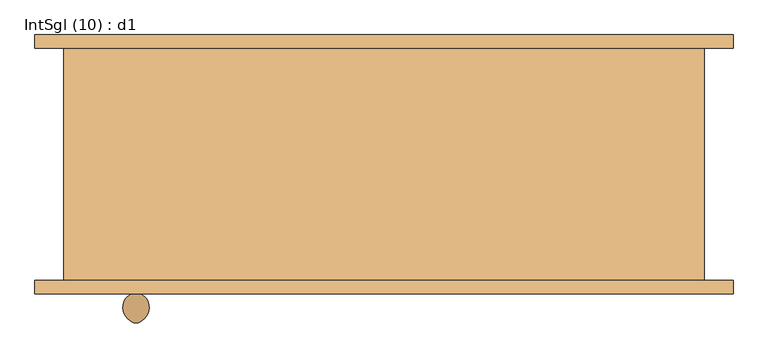
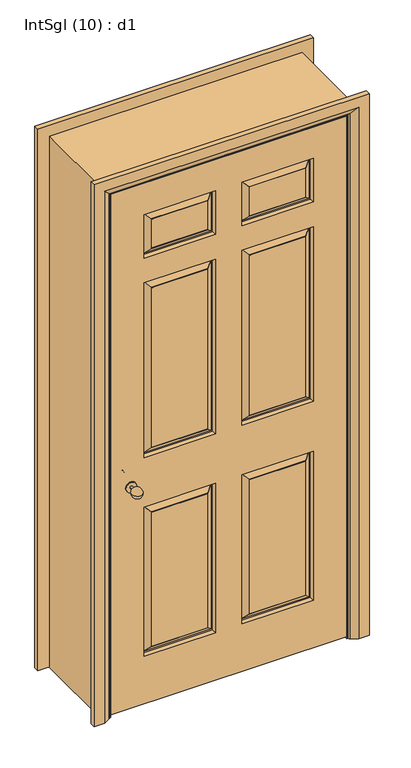
"""IFC4 building model written with IfcOpenShell, lengths in millimetres: door geometry, IntSgl (10) : d1."""

from ifc_helpers import new_model, si_unit, point, frame, origin, place, context, project, spatial, polyline, circle_curve, ellipse_curve, trimmed, outline, extrude, faceted_brep, source, transform, mapped, element, save
from ifc_brep_helpers import plane_surface, cylinder_surface, revolved_surface, advanced_brep


def intsgl_10_d1_80eab747(model_context):
    return source(origin(), model_context, "Body", "SolidModel", [
        advanced_brep(
        [(-368.0, -118.0, 900.0), (-378.0, -118.0, 900.0), (-373.0, -73.562589, 900.0), (-368.0, -133.0, 900.0), (-378.0, -133.0, 900.0), (-393.0, -137.0, 900.0), (-353.0, -137.0, 900.0), (-393.0, -133.0, 900.0), (-353.0, -133.0, 900.0)],
        [
            (0, 1, circle_curve(frame((-373.0, -118.0, 900.0), z_axis=(0.0, 1.0, 0.0), x_axis=(-1.0, 0.0, 0.0)), 5.0)),
            (1, 2, circle_curve(frame((-369.8115138, -96.4213505, 900.0), z_axis=(0.0, 0.0, -1.0), x_axis=(0.0, -1.0, 0.0)), 23.0800654)),
            (2, 0, circle_curve(frame((-376.1884862, -96.4213505, 900.0), z_axis=(0.0, 0.0, -1.0), x_axis=(0.0, -1.0, 0.0)), 23.0800654)),
            (1, 0, circle_curve(frame((-373.0, -118.0, 900.0), z_axis=(0.0, 1.0, 0.0), x_axis=(-1.0, 0.0, 0.0)), 5.0)),
            (0, 3),
            (3, 4, circle_curve(frame((-373.0, -133.0, 900.0), z_axis=(0.0, 1.0, 0.0), x_axis=(-1.0, 0.0, 0.0)), 5.0)),
            (4, 1),
            (4, 3, circle_curve(frame((-373.0, -133.0, 900.0), z_axis=(0.0, 1.0, 0.0), x_axis=(-1.0, 0.0, 0.0)), 5.0)),
            (5, 6, circle_curve(frame((-373.0, -137.0, 900.0), z_axis=(0.0, -1.0, 0.0), x_axis=(1.0, 0.0, 0.0)), 20.0)),
            (6, 5, circle_curve(frame((-373.0, -137.0, 900.0), z_axis=(0.0, -1.0, 0.0), x_axis=(1.0, 0.0, 0.0)), 20.0)),
            (7, 8, circle_curve(frame((-373.0, -133.0, 900.0), z_axis=(0.0, 1.0, 0.0), x_axis=(1.0, 0.0, 0.0)), 20.0)),
            (8, 7, circle_curve(frame((-373.0, -133.0, 900.0), z_axis=(0.0, 1.0, 0.0), x_axis=(1.0, 0.0, 0.0)), 20.0)),
            (5, 7),
            (8, 6),
        ],
        [
            revolved_surface(trimmed(ellipse_curve(frame((-369.8115138, -96.4213505, 900.0), z_axis=(0.0, 0.0, 1.0), x_axis=(0.0, -1.0, 0.0)), 23.0800654, 23.0800654), [point((-373.0, -73.562589, 900.0))], [point((-378.0, -118.0, 900.0))], True, "CARTESIAN"), (-373.0, -133.0, 900.0), (0.0, -1.0, 0.0)),
            cylinder_surface(frame((-373.0, -133.0, 900.0), z_axis=(0.0, -1.0, 0.0), x_axis=(-1.0, 0.0, 0.0)), 5.0),
            plane_surface(frame((-353.0, -137.0, 900.0), z_axis=(0.0, -1.0, 0.0), x_axis=(0.0, 0.0, 1.0))),
            plane_surface(frame((-353.0, -133.0, 900.0), z_axis=(0.0, 1.0, 0.0), x_axis=(0.0, 0.0, -1.0))),
            cylinder_surface(frame((-373.0, -133.0, 900.0), z_axis=(0.0, -1.0, 0.0), x_axis=(1.0, 0.0, 0.0)), 20.0),
        ],
        [
            (0, [[1, 2, 3]]),
            (0, [[-2, 4, -3]]),
            (1, [[-1, 5, 6, 7]]),
            (1, [[-4, -7, 8, -5]]),
            (2, [[9, 10]]),
            (3, [[11, 12], [-6, -8]]),
            (4, [[-9, 13, -12, 14]]),
            (4, [[-10, -14, -11, -13]]),
        ],
    ),
        advanced_brep(
        [(-368.0, -194.0, 900.0), (-373.0, -238.437411, 900.0), (-378.0, -194.0, 900.0), (-378.0, -179.0, 900.0), (-368.0, -179.0, 900.0), (-393.0, -175.0, 900.0), (-353.0, -175.0, 900.0), (-393.0, -179.0, 900.0), (-353.0, -179.0, 900.0)],
        [
            (0, 1, circle_curve(frame((-376.1884862, -215.5786495, 900.0), z_axis=(0.0, 0.0, -1.0), x_axis=(0.0, 1.0, 0.0)), 23.0800654)),
            (1, 2, circle_curve(frame((-369.8115138, -215.5786495, 900.0), z_axis=(0.0, 0.0, -1.0), x_axis=(0.0, 1.0, 0.0)), 23.0800654)),
            (2, 0, circle_curve(frame((-373.0, -194.0, 900.0), z_axis=(0.0, -1.0, 0.0), x_axis=(-1.0, 0.0, 0.0)), 5.0)),
            (0, 2, circle_curve(frame((-373.0, -194.0, 900.0), z_axis=(0.0, -1.0, 0.0), x_axis=(-1.0, 0.0, 0.0)), 5.0)),
            (2, 3),
            (3, 4, circle_curve(frame((-373.0, -179.0, 900.0), z_axis=(0.0, -1.0, 0.0), x_axis=(-1.0, 0.0, 0.0)), 5.0)),
            (4, 0),
            (4, 3, circle_curve(frame((-373.0, -179.0, 900.0), z_axis=(0.0, -1.0, 0.0), x_axis=(-1.0, 0.0, 0.0)), 5.0)),
            (5, 6, circle_curve(frame((-373.0, -175.0, 900.0), z_axis=(0.0, 1.0, 0.0), x_axis=(1.0, 0.0, 0.0)), 20.0)),
            (6, 5, circle_curve(frame((-373.0, -175.0, 900.0), z_axis=(0.0, 1.0, 0.0), x_axis=(1.0, 0.0, 0.0)), 20.0)),
            (7, 8, circle_curve(frame((-373.0, -179.0, 900.0), z_axis=(0.0, -1.0, 0.0), x_axis=(1.0, 0.0, 0.0)), 20.0)),
            (8, 7, circle_curve(frame((-373.0, -179.0, 900.0), z_axis=(0.0, -1.0, 0.0), x_axis=(1.0, 0.0, 0.0)), 20.0)),
            (6, 8),
            (7, 5),
        ],
        [
            revolved_surface(trimmed(ellipse_curve(frame((-369.8115138, -215.5786495, 900.0), z_axis=(0.0, 0.0, -1.0), x_axis=(0.0, 1.0, 0.0)), 23.0800654, 23.0800654), [point((-373.0, -238.437411, 900.0))], [point((-378.0, -194.0, 900.0))], True, "CARTESIAN"), (-373.0, -179.0, 900.0), (0.0, 1.0, 0.0)),
            cylinder_surface(frame((-373.0, -179.0, 900.0), z_axis=(0.0, 1.0, 0.0), x_axis=(-1.0, 0.0, 0.0)), 5.0),
            plane_surface(frame((-353.0, -175.0, 900.0), z_axis=(0.0, 1.0, 0.0), x_axis=(0.0, 0.0, 1.0))),
            plane_surface(frame((-353.0, -179.0, 900.0), z_axis=(0.0, -1.0, 0.0), x_axis=(0.0, 0.0, -1.0))),
            cylinder_surface(frame((-373.0, -179.0, 900.0), z_axis=(0.0, 1.0, 0.0), x_axis=(1.0, 0.0, 0.0)), 20.0),
        ],
        [
            (0, [[1, 2, 3]]),
            (0, [[-1, 4, -2]]),
            (1, [[5, 6, 7, -3]]),
            (1, [[-7, 8, -5, -4]]),
            (2, [[9, 10]]),
            (3, [[11, 12], [-8, -6]]),
            (4, [[13, -11, 14, -10]]),
            (4, [[-14, -12, -13, -9]]),
        ],
    ),
        faceted_brep([(-448.0, -137.0, 2103.0), (448.0, -137.0, 2103.0), (448.0, -137.0, 8.0), (-448.0, -137.0, 8.0), (-50.0, -137.0, 800.0), (-323.0, -137.0, 800.0), (-323.0, -137.0, 200.0), (-50.0, -137.0, 200.0), (323.0, -137.0, 800.0), (50.0, -137.0, 800.0), (50.0, -137.0, 200.0), (323.0, -137.0, 200.0), (-50.0, -137.0, 1703.0), (-323.0, -137.0, 1703.0), (-323.0, -137.0, 1000.0), (-50.0, -137.0, 1000.0), (323.0, -137.0, 1703.0), (50.0, -137.0, 1703.0), (50.0, -137.0, 1000.0), (323.0, -137.0, 1000.0), (-50.0, -137.0, 1978.0), (-323.0, -137.0, 1978.0), (-323.0, -137.0, 1803.0), (-50.0, -137.0, 1803.0), (323.0, -137.0, 1978.0), (50.0, -137.0, 1978.0), (50.0, -137.0, 1803.0), (323.0, -137.0, 1803.0), (-80.0, -137.0, 230.0), (-293.0, -137.0, 230.0), (-293.0, -137.0, 770.0), (-80.0, -137.0, 770.0), (293.0, -137.0, 230.0), (80.0, -137.0, 230.0), (80.0, -137.0, 770.0), (293.0, -137.0, 770.0), (-80.0, -137.0, 1030.0), (-293.0, -137.0, 1030.0), (-293.0, -137.0, 1673.0), (-80.0, -137.0, 1673.0), (293.0, -137.0, 1030.0), (80.0, -137.0, 1030.0), (80.0, -137.0, 1673.0), (293.0, -137.0, 1673.0), (-80.0, -137.0, 1833.0), (-293.0, -137.0, 1833.0), (-293.0, -137.0, 1948.0), (-80.0, -137.0, 1948.0), (293.0, -137.0, 1833.0), (80.0, -137.0, 1833.0), (80.0, -137.0, 1948.0), (293.0, -137.0, 1948.0), (-448.0, -175.0, 2103.0), (-448.0, -175.0, 8.0), (448.0, -175.0, 8.0), (448.0, -175.0, 2103.0), (50.0, -175.0, 800.0), (323.0, -175.0, 800.0), (323.0, -175.0, 200.0), (50.0, -175.0, 200.0), (-323.0, -175.0, 800.0), (-50.0, -175.0, 800.0), (-50.0, -175.0, 200.0), (-323.0, -175.0, 200.0), (50.0, -175.0, 1703.0), (323.0, -175.0, 1703.0), (323.0, -175.0, 1000.0), (50.0, -175.0, 1000.0), (-323.0, -175.0, 1703.0), (-50.0, -175.0, 1703.0), (-50.0, -175.0, 1000.0), (-323.0, -175.0, 1000.0), (50.0, -175.0, 1978.0), (323.0, -175.0, 1978.0), (323.0, -175.0, 1803.0), (50.0, -175.0, 1803.0), (-323.0, -175.0, 1978.0), (-50.0, -175.0, 1978.0), (-50.0, -175.0, 1803.0), (-323.0, -175.0, 1803.0), (80.0, -175.0, 230.0), (293.0, -175.0, 230.0), (293.0, -175.0, 770.0), (80.0, -175.0, 770.0), (-293.0, -175.0, 230.0), (-80.0, -175.0, 230.0), (-80.0, -175.0, 770.0), (-293.0, -175.0, 770.0), (80.0, -175.0, 1030.0), (293.0, -175.0, 1030.0), (293.0, -175.0, 1673.0), (80.0, -175.0, 1673.0), (-293.0, -175.0, 1030.0), (-80.0, -175.0, 1030.0), (-80.0, -175.0, 1673.0), (-293.0, -175.0, 1673.0), (80.0, -175.0, 1833.0), (293.0, -175.0, 1833.0), (293.0, -175.0, 1948.0), (80.0, -175.0, 1948.0), (-293.0, -175.0, 1833.0), (-80.0, -175.0, 1833.0), (-80.0, -175.0, 1948.0), (-293.0, -175.0, 1948.0), (80.0, -174.0, 230.0), (80.0, -174.0, 770.0), (58.0, -160.0, 208.0), (78.0, -174.0, 228.0), (78.0, -174.0, 772.0), (58.0, -160.0, 792.0), (53.0, -160.0, 203.0), (53.0, -160.0, 797.0), (293.0, -174.0, 770.0), (295.0, -174.0, 772.0), (315.0, -160.0, 792.0), (320.0, -160.0, 797.0), (293.0, -174.0, 230.0), (295.0, -174.0, 228.0), (315.0, -160.0, 208.0), (320.0, -160.0, 203.0), (-293.0, -174.0, 230.0), (-293.0, -174.0, 770.0), (-315.0, -160.0, 208.0), (-295.0, -174.0, 228.0), (-295.0, -174.0, 772.0), (-315.0, -160.0, 792.0), (-320.0, -160.0, 203.0), (-320.0, -160.0, 797.0), (-80.0, -174.0, 770.0), (-78.0, -174.0, 772.0), (-58.0, -160.0, 792.0), (-53.0, -160.0, 797.0), (-80.0, -174.0, 230.0), (-78.0, -174.0, 228.0), (-58.0, -160.0, 208.0), (-53.0, -160.0, 203.0), (80.0, -174.0, 1030.0), (80.0, -174.0, 1673.0), (58.0, -160.0, 1008.0), (78.0, -174.0, 1028.0), (78.0, -174.0, 1675.0), (58.0, -160.0, 1695.0), (53.0, -160.0, 1003.0), (53.0, -160.0, 1700.0), (293.0, -174.0, 1673.0), (295.0, -174.0, 1675.0), (315.0, -160.0, 1695.0), (320.0, -160.0, 1700.0), (293.0, -174.0, 1030.0), (295.0, -174.0, 1028.0), (315.0, -160.0, 1008.0), (320.0, -160.0, 1003.0), (-293.0, -174.0, 1030.0), (-293.0, -174.0, 1673.0), (-315.0, -160.0, 1008.0), (-295.0, -174.0, 1028.0), (-295.0, -174.0, 1675.0), (-315.0, -160.0, 1695.0), (-320.0, -160.0, 1003.0), (-320.0, -160.0, 1700.0), (-80.0, -174.0, 1673.0), (-78.0, -174.0, 1675.0), (-58.0, -160.0, 1695.0), (-53.0, -160.0, 1700.0), (-80.0, -174.0, 1030.0), (-78.0, -174.0, 1028.0), (-58.0, -160.0, 1008.0), (-53.0, -160.0, 1003.0), (80.0, -174.0, 1833.0), (80.0, -174.0, 1948.0), (58.0, -160.0, 1811.0), (78.0, -174.0, 1831.0), (78.0, -174.0, 1950.0), (58.0, -160.0, 1970.0), (53.0, -160.0, 1806.0), (53.0, -160.0, 1975.0), (293.0, -174.0, 1948.0), (295.0, -174.0, 1950.0), (315.0, -160.0, 1970.0), (320.0, -160.0, 1975.0), (293.0, -174.0, 1833.0), (295.0, -174.0, 1831.0), (315.0, -160.0, 1811.0), (320.0, -160.0, 1806.0), (-293.0, -174.0, 1833.0), (-293.0, -174.0, 1948.0), (-315.0, -160.0, 1811.0), (-295.0, -174.0, 1831.0), (-295.0, -174.0, 1950.0), (-315.0, -160.0, 1970.0), (-320.0, -160.0, 1806.0), (-320.0, -160.0, 1975.0), (-80.0, -174.0, 1948.0), (-78.0, -174.0, 1950.0), (-58.0, -160.0, 1970.0), (-53.0, -160.0, 1975.0), (-80.0, -174.0, 1833.0), (-78.0, -174.0, 1831.0), (-58.0, -160.0, 1811.0), (-53.0, -160.0, 1806.0), (-80.0, -138.0, 230.0), (-80.0, -138.0, 770.0), (-58.0, -152.0, 208.0), (-78.0, -138.0, 228.0), (-78.0, -138.0, 772.0), (-58.0, -152.0, 792.0), (-53.0, -152.0, 203.0), (-53.0, -152.0, 797.0), (-293.0, -138.0, 770.0), (-295.0, -138.0, 772.0), (-315.0, -152.0, 792.0), (-320.0, -152.0, 797.0), (-293.0, -138.0, 230.0), (-295.0, -138.0, 228.0), (-315.0, -152.0, 208.0), (-320.0, -152.0, 203.0), (293.0, -138.0, 230.0), (293.0, -138.0, 770.0), (315.0, -152.0, 208.0), (295.0, -138.0, 228.0), (295.0, -138.0, 772.0), (315.0, -152.0, 792.0), (320.0, -152.0, 203.0), (320.0, -152.0, 797.0), (80.0, -138.0, 770.0), (78.0, -138.0, 772.0), (58.0, -152.0, 792.0), (53.0, -152.0, 797.0), (80.0, -138.0, 230.0), (78.0, -138.0, 228.0), (58.0, -152.0, 208.0), (53.0, -152.0, 203.0), (-80.0, -138.0, 1030.0), (-80.0, -138.0, 1673.0), (-58.0, -152.0, 1008.0), (-78.0, -138.0, 1028.0), (-78.0, -138.0, 1675.0), (-58.0, -152.0, 1695.0), (-53.0, -152.0, 1003.0), (-53.0, -152.0, 1700.0), (-293.0, -138.0, 1673.0), (-295.0, -138.0, 1675.0), (-315.0, -152.0, 1695.0), (-320.0, -152.0, 1700.0), (-293.0, -138.0, 1030.0), (-295.0, -138.0, 1028.0), (-315.0, -152.0, 1008.0), (-320.0, -152.0, 1003.0), (293.0, -138.0, 1030.0), (293.0, -138.0, 1673.0), (315.0, -152.0, 1008.0), (295.0, -138.0, 1028.0), (295.0, -138.0, 1675.0), (315.0, -152.0, 1695.0), (320.0, -152.0, 1003.0), (320.0, -152.0, 1700.0), (80.0, -138.0, 1673.0), (78.0, -138.0, 1675.0), (58.0, -152.0, 1695.0), (53.0, -152.0, 1700.0), (80.0, -138.0, 1030.0), (78.0, -138.0, 1028.0), (58.0, -152.0, 1008.0), (53.0, -152.0, 1003.0), (-80.0, -138.0, 1833.0), (-80.0, -138.0, 1948.0), (-58.0, -152.0, 1811.0), (-78.0, -138.0, 1831.0), (-78.0, -138.0, 1950.0), (-58.0, -152.0, 1970.0), (-53.0, -152.0, 1806.0), (-53.0, -152.0, 1975.0), (-293.0, -138.0, 1948.0), (-295.0, -138.0, 1950.0), (-315.0, -152.0, 1970.0), (-320.0, -152.0, 1975.0), (-293.0, -138.0, 1833.0), (-295.0, -138.0, 1831.0), (-315.0, -152.0, 1811.0), (-320.0, -152.0, 1806.0), (293.0, -138.0, 1833.0), (293.0, -138.0, 1948.0), (315.0, -152.0, 1811.0), (295.0, -138.0, 1831.0), (295.0, -138.0, 1950.0), (315.0, -152.0, 1970.0), (320.0, -152.0, 1806.0), (320.0, -152.0, 1975.0), (80.0, -138.0, 1948.0), (78.0, -138.0, 1950.0), (58.0, -152.0, 1970.0), (53.0, -152.0, 1975.0), (80.0, -138.0, 1833.0), (78.0, -138.0, 1831.0), (58.0, -152.0, 1811.0), (53.0, -152.0, 1806.0)], [[[0, 1, 2, 3], [4, 5, 6, 7], [8, 9, 10, 11], [12, 13, 14, 15], [16, 17, 18, 19], [20, 21, 22, 23], [24, 25, 26, 27]], [[28, 29, 30, 31]], [[32, 33, 34, 35]], [[36, 37, 38, 39]], [[40, 41, 42, 43]], [[44, 45, 46, 47]], [[48, 49, 50, 51]], [[52, 53, 54, 55], [56, 57, 58, 59], [60, 61, 62, 63], [64, 65, 66, 67], [68, 69, 70, 71], [72, 73, 74, 75], [76, 77, 78, 79]], [[80, 81, 82, 83]], [[84, 85, 86, 87]], [[88, 89, 90, 91]], [[92, 93, 94, 95]], [[96, 97, 98, 99]], [[100, 101, 102, 103]], [[3, 53, 52, 0]], [[2, 54, 53, 3]], [[1, 55, 54, 2]], [[0, 52, 55, 1]], [[104, 80, 83, 105]], [[106, 107, 108, 109]], [[56, 59, 110, 111]], [[83, 82, 112, 105]], [[108, 113, 114, 109]], [[111, 115, 57, 56]], [[82, 81, 116, 112]], [[113, 117, 118, 114]], [[115, 119, 58, 57]], [[104, 116, 81, 80]], [[107, 117, 113, 108], [105, 112, 116, 104]], [[106, 118, 117, 107]], [[110, 119, 115, 111], [109, 114, 118, 106]], [[59, 58, 119, 110]], [[120, 84, 87, 121]], [[122, 123, 124, 125]], [[60, 63, 126, 127]], [[87, 86, 128, 121]], [[124, 129, 130, 125]], [[127, 131, 61, 60]], [[86, 85, 132, 128]], [[129, 133, 134, 130]], [[131, 135, 62, 61]], [[120, 132, 85, 84]], [[123, 133, 129, 124], [121, 128, 132, 120]], [[122, 134, 133, 123]], [[126, 135, 131, 127], [125, 130, 134, 122]], [[63, 62, 135, 126]], [[136, 88, 91, 137]], [[138, 139, 140, 141]], [[64, 67, 142, 143]], [[91, 90, 144, 137]], [[140, 145, 146, 141]], [[143, 147, 65, 64]], [[90, 89, 148, 144]], [[145, 149, 150, 146]], [[147, 151, 66, 65]], [[136, 148, 89, 88]], [[139, 149, 145, 140], [137, 144, 148, 136]], [[138, 150, 149, 139]], [[142, 151, 147, 143], [141, 146, 150, 138]], [[67, 66, 151, 142]], [[152, 92, 95, 153]], [[154, 155, 156, 157]], [[68, 71, 158, 159]], [[95, 94, 160, 153]], [[156, 161, 162, 157]], [[159, 163, 69, 68]], [[94, 93, 164, 160]], [[161, 165, 166, 162]], [[163, 167, 70, 69]], [[152, 164, 93, 92]], [[155, 165, 161, 156], [153, 160, 164, 152]], [[154, 166, 165, 155]], [[158, 167, 163, 159], [157, 162, 166, 154]], [[71, 70, 167, 158]], [[168, 96, 99, 169]], [[170, 171, 172, 173]], [[72, 75, 174, 175]], [[99, 98, 176, 169]], [[172, 177, 178, 173]], [[175, 179, 73, 72]], [[98, 97, 180, 176]], [[177, 181, 182, 178]], [[179, 183, 74, 73]], [[168, 180, 97, 96]], [[171, 181, 177, 172], [169, 176, 180, 168]], [[170, 182, 181, 171]], [[174, 183, 179, 175], [173, 178, 182, 170]], [[75, 74, 183, 174]], [[184, 100, 103, 185]], [[186, 187, 188, 189]], [[76, 79, 190, 191]], [[103, 102, 192, 185]], [[188, 193, 194, 189]], [[191, 195, 77, 76]], [[102, 101, 196, 192]], [[193, 197, 198, 194]], [[195, 199, 78, 77]], [[184, 196, 101, 100]], [[187, 197, 193, 188], [185, 192, 196, 184]], [[186, 198, 197, 187]], [[190, 199, 195, 191], [189, 194, 198, 186]], [[79, 78, 199, 190]], [[200, 28, 31, 201]], [[202, 203, 204, 205]], [[4, 7, 206, 207]], [[31, 30, 208, 201]], [[204, 209, 210, 205]], [[207, 211, 5, 4]], [[30, 29, 212, 208]], [[209, 213, 214, 210]], [[211, 215, 6, 5]], [[200, 212, 29, 28]], [[203, 213, 209, 204], [201, 208, 212, 200]], [[202, 214, 213, 203]], [[206, 215, 211, 207], [205, 210, 214, 202]], [[7, 6, 215, 206]], [[216, 32, 35, 217]], [[218, 219, 220, 221]], [[8, 11, 222, 223]], [[35, 34, 224, 217]], [[220, 225, 226, 221]], [[223, 227, 9, 8]], [[34, 33, 228, 224]], [[225, 229, 230, 226]], [[227, 231, 10, 9]], [[216, 228, 33, 32]], [[219, 229, 225, 220], [217, 224, 228, 216]], [[218, 230, 229, 219]], [[222, 231, 227, 223], [221, 226, 230, 218]], [[11, 10, 231, 222]], [[232, 36, 39, 233]], [[234, 235, 236, 237]], [[12, 15, 238, 239]], [[39, 38, 240, 233]], [[236, 241, 242, 237]], [[239, 243, 13, 12]], [[38, 37, 244, 240]], [[241, 245, 246, 242]], [[243, 247, 14, 13]], [[232, 244, 37, 36]], [[235, 245, 241, 236], [233, 240, 244, 232]], [[234, 246, 245, 235]], [[238, 247, 243, 239], [237, 242, 246, 234]], [[15, 14, 247, 238]], [[248, 40, 43, 249]], [[250, 251, 252, 253]], [[16, 19, 254, 255]], [[43, 42, 256, 249]], [[252, 257, 258, 253]], [[255, 259, 17, 16]], [[42, 41, 260, 256]], [[257, 261, 262, 258]], [[259, 263, 18, 17]], [[248, 260, 41, 40]], [[251, 261, 257, 252], [249, 256, 260, 248]], [[250, 262, 261, 251]], [[254, 263, 259, 255], [253, 258, 262, 250]], [[19, 18, 263, 254]], [[264, 44, 47, 265]], [[266, 267, 268, 269]], [[20, 23, 270, 271]], [[47, 46, 272, 265]], [[268, 273, 274, 269]], [[271, 275, 21, 20]], [[46, 45, 276, 272]], [[273, 277, 278, 274]], [[275, 279, 22, 21]], [[264, 276, 45, 44]], [[267, 277, 273, 268], [265, 272, 276, 264]], [[266, 278, 277, 267]], [[270, 279, 275, 271], [269, 274, 278, 266]], [[23, 22, 279, 270]], [[280, 48, 51, 281]], [[282, 283, 284, 285]], [[24, 27, 286, 287]], [[51, 50, 288, 281]], [[284, 289, 290, 285]], [[287, 291, 25, 24]], [[50, 49, 292, 288]], [[289, 293, 294, 290]], [[291, 295, 26, 25]], [[280, 292, 49, 48]], [[283, 293, 289, 284], [281, 288, 292, 280]], [[282, 294, 293, 283]], [[286, 295, 291, 287], [285, 290, 294, 282]], [[27, 26, 295, 286]]]),
        advanced_brep(
        [(525.0, -195.0, 0.0), (485.0, -195.0, 0.0), (459.0, -181.0, 0.0), (455.0, -175.0, 0.0), (525.0, -175.0, 0.0), (525.0, -175.0, 2180.0), (525.0, -195.0, 2180.0), (455.0, -175.0, 2110.0), (-455.0, -175.0, 2110.0), (-455.0, -175.0, 0.0), (-525.0, -175.0, 0.0), (-525.0, -175.0, 2180.0), (459.0, -181.0, 2114.0), (485.0, -195.0, 2140.0), (-525.0, -195.0, 2180.0), (-525.0, -195.0, 0.0), (-485.0, -195.0, 0.0), (-485.0, -195.0, 2140.0), (-459.0, -181.0, 0.0), (-459.0, -181.0, 2114.0)],
        [
            (0, 1),
            (1, 2),
            (2, 3, circle_curve(frame((463.0, -174.0, 0.0), z_axis=(0.0, 0.0, -1.0), x_axis=(1.0, 0.0, 0.0)), 8.0622577)),
            (3, 4),
            (4, 0),
            (4, 5),
            (5, 6),
            (6, 0),
            (3, 7),
            (7, 8),
            (8, 9),
            (9, 10),
            (10, 11),
            (11, 5),
            (2, 12),
            (12, 7, ellipse_curve(frame((463.0, -174.0, 2118.0), z_axis=(0.7071067811865475, 0.0, -0.7071067811865475), x_axis=(-0.7071067811865474, 0.0, -0.7071067811865476)), 11.4017543, 8.0622577)),
            (1, 13),
            (13, 12),
            (6, 14),
            (14, 15),
            (15, 16),
            (16, 17),
            (17, 13),
            (10, 15),
            (14, 11),
            (9, 18, circle_curve(frame((-463.0, -174.0, 0.0), z_axis=(0.0, 0.0, -1.0), x_axis=(-1.0, 0.0, 0.0)), 8.0622577)),
            (18, 16),
            (19, 18),
            (8, 19, ellipse_curve(frame((-463.0, -174.0, 2118.0), z_axis=(-0.7071067811865475, 0.0, -0.7071067811865475), x_axis=(-0.7071067811865474, 0.0, 0.7071067811865476)), 11.4017543, 8.0622577)),
            (19, 17),
            (12, 19),
        ],
        [
            plane_surface(frame((455.0, -175.0, 0.0), z_axis=(0.0, 0.0, -1.0), x_axis=(0.0, -1.0, 0.0))),
            plane_surface(frame((525.0, -195.0, 0.0), z_axis=(1.0, 0.0, 0.0), x_axis=(0.0, 0.0, 1.0))),
            plane_surface(frame((525.0, -175.0, 0.0), z_axis=(0.0, 1.0, 0.0), x_axis=(0.0, 0.0, 1.0))),
            cylinder_surface(frame((463.0, -174.0, 0.0), z_axis=(0.0, 0.0, -1.0), x_axis=(1.0, 0.0, 0.0)), 8.0622577),
            plane_surface(frame((459.0, -181.0, 0.0), z_axis=(-0.4740998230350183, -0.8804710999221749, 0.0), x_axis=(0.0, 0.0, 1.0))),
            plane_surface(frame((485.0, -195.0, 0.0), z_axis=(0.0, -1.0, 0.0), x_axis=(0.0, 0.0, 1.0))),
            plane_surface(frame((-525.0, -195.0, 2180.0), z_axis=(-1.0, 0.0, 0.0), x_axis=(0.0, 0.0, -1.0))),
            plane_surface(frame((-455.0, -175.0, 0.0), z_axis=(0.0, 0.0, -1.0), x_axis=(0.0, -1.0, 0.0))),
            cylinder_surface(frame((-463.0, -174.0, 2110.0), z_axis=(0.0, 0.0, 1.0), x_axis=(-1.0, 0.0, 0.0)), 8.0622577),
            plane_surface(frame((-459.0, -181.0, 2114.0), z_axis=(0.4740998230350183, -0.8804710999221749, 0.0), x_axis=(0.0, 0.0, -1.0))),
            plane_surface(frame((525.0, -195.0, 2180.0), z_axis=(0.0, 0.0, 1.0), x_axis=(-1.0, 0.0, 0.0))),
            cylinder_surface(frame((455.0, -174.0, 2118.0), z_axis=(1.0, 0.0, 0.0), x_axis=(0.0, 0.0, 1.0)), 8.0622577),
            plane_surface(frame((459.0, -181.0, 2114.0), z_axis=(0.0, -0.8804710999221749, -0.4740998230350183), x_axis=(-1.0, 0.0, 0.0))),
        ],
        [
            (0, [[1, 2, 3, 4, 5]]),
            (1, [[6, 7, 8, -5]]),
            (2, [[9, 10, 11, 12, 13, 14, -6, -4]]),
            (3, [[15, 16, -9, -3]]),
            (4, [[17, 18, -15, -2]]),
            (5, [[-8, 19, 20, 21, 22, 23, -17, -1]]),
            (6, [[-13, 24, -20, 25]]),
            (7, [[-24, -12, 26, 27, -21]]),
            (8, [[28, -26, -11, 29]]),
            (9, [[-22, -27, -28, 30]]),
            (10, [[-14, -25, -19, -7]]),
            (11, [[31, -29, -10, -16]]),
            (12, [[-23, -30, -31, -18]]),
        ],
    ),
        advanced_brep(
        [(-525.0, 195.0, 0.0), (-485.0, 195.0, 0.0), (-459.0, 181.0, 0.0), (-455.0, 175.0, 0.0), (-525.0, 175.0, 0.0), (-525.0, 175.0, 2180.0), (-525.0, 195.0, 2180.0), (-455.0, 175.0, 2110.0), (455.0, 175.0, 2110.0), (455.0, 175.0, 0.0), (525.0, 175.0, 0.0), (525.0, 175.0, 2180.0), (-459.0, 181.0, 2114.0), (-485.0, 195.0, 2140.0), (525.0, 195.0, 2180.0), (525.0, 195.0, 0.0), (485.0, 195.0, 0.0), (485.0, 195.0, 2140.0), (459.0, 181.0, 0.0), (459.0, 181.0, 2114.0)],
        [
            (0, 1),
            (1, 2),
            (2, 3, circle_curve(frame((-463.0, 174.0, 0.0), z_axis=(0.0, 0.0, -1.0), x_axis=(-1.0, 0.0, 0.0)), 8.0622577)),
            (3, 4),
            (4, 0),
            (4, 5),
            (5, 6),
            (6, 0),
            (3, 7),
            (7, 8),
            (8, 9),
            (9, 10),
            (10, 11),
            (11, 5),
            (2, 12),
            (12, 7, ellipse_curve(frame((-463.0, 174.0, 2118.0), z_axis=(-0.7071067811865475, 0.0, -0.7071067811865475), x_axis=(0.7071067811865474, 0.0, -0.7071067811865476)), 11.4017543, 8.0622577)),
            (1, 13),
            (13, 12),
            (6, 14),
            (14, 15),
            (15, 16),
            (16, 17),
            (17, 13),
            (10, 15),
            (14, 11),
            (9, 18, circle_curve(frame((463.0, 174.0, 0.0), z_axis=(0.0, 0.0, -1.0), x_axis=(1.0, 0.0, 0.0)), 8.0622577)),
            (18, 16),
            (19, 18),
            (8, 19, ellipse_curve(frame((463.0, 174.0, 2118.0), z_axis=(0.7071067811865475, 0.0, -0.7071067811865475), x_axis=(0.7071067811865474, 0.0, 0.7071067811865476)), 11.4017543, 8.0622577)),
            (19, 17),
            (12, 19),
        ],
        [
            plane_surface(frame((-455.0, 175.0, 0.0), z_axis=(0.0, 0.0, -1.0), x_axis=(0.0, 1.0, 0.0))),
            plane_surface(frame((-525.0, 195.0, 0.0), z_axis=(-1.0, 0.0, 0.0), x_axis=(0.0, 0.0, 1.0))),
            plane_surface(frame((-525.0, 175.0, 0.0), z_axis=(0.0, -1.0, 0.0), x_axis=(0.0, 0.0, 1.0))),
            cylinder_surface(frame((-463.0, 174.0, 0.0), z_axis=(0.0, 0.0, -1.0), x_axis=(-1.0, 0.0, 0.0)), 8.0622577),
            plane_surface(frame((-459.0, 181.0, 0.0), z_axis=(0.4740998230350183, 0.8804710999221749, 0.0), x_axis=(0.0, 0.0, 1.0))),
            plane_surface(frame((-485.0, 195.0, 0.0), z_axis=(0.0, 1.0, 0.0), x_axis=(0.0, 0.0, 1.0))),
            plane_surface(frame((525.0, 195.0, 2180.0), z_axis=(1.0, 0.0, 0.0), x_axis=(0.0, 0.0, -1.0))),
            plane_surface(frame((455.0, 175.0, 0.0), z_axis=(0.0, 0.0, -1.0), x_axis=(0.0, 1.0, 0.0))),
            cylinder_surface(frame((463.0, 174.0, 2110.0), z_axis=(0.0, 0.0, 1.0), x_axis=(1.0, 0.0, 0.0)), 8.0622577),
            plane_surface(frame((459.0, 181.0, 2114.0), z_axis=(-0.4740998230350183, 0.8804710999221749, 0.0), x_axis=(0.0, 0.0, -1.0))),
            plane_surface(frame((-525.0, 195.0, 2180.0), z_axis=(0.0, 0.0, 1.0), x_axis=(1.0, 0.0, 0.0))),
            cylinder_surface(frame((-455.0, 174.0, 2118.0), z_axis=(-1.0, 0.0, 0.0), x_axis=(0.0, 0.0, 1.0)), 8.0622577),
            plane_surface(frame((-459.0, 181.0, 2114.0), z_axis=(0.0, 0.8804710999221749, -0.4740998230350183), x_axis=(1.0, 0.0, 0.0))),
        ],
        [
            (0, [[1, 2, 3, 4, 5]]),
            (1, [[6, 7, 8, -5]]),
            (2, [[9, 10, 11, 12, 13, 14, -6, -4]]),
            (3, [[15, 16, -9, -3]]),
            (4, [[17, 18, -15, -2]]),
            (5, [[-8, 19, 20, 21, 22, 23, -17, -1]]),
            (6, [[-13, 24, -20, 25]]),
            (7, [[-24, -12, 26, 27, -21]]),
            (8, [[28, -26, -11, 29]]),
            (9, [[-22, -27, -28, 30]]),
            (10, [[-14, -25, -19, -7]]),
            (11, [[31, -29, -10, -16]]),
            (12, [[-23, -30, -31, -18]]),
        ],
    ),
        extrude(outline(polyline([(0.0, -431.0), (2086.0, -431.0), (2086.0, 431.0), (0.0, 431.0), (0.0, 450.0), (2105.0, 450.0), (2105.0, -450.0), (0.0, -450.0), (0.0, -431.0)])), frame((0.0, -135.0, 0.0), z_axis=(0.0, 1.0, 0.0), x_axis=(0.0, 0.0, 1.0)), (0.0, 0.0, 1.0), 32.0),
        faceted_brep([(-450.0, -175.0, 0.0), (-482.0, -175.0, 0.0), (-482.0, 175.0, 0.0), (-450.0, 175.0, 0.0), (-450.0, 175.0, 2105.0), (-450.0, -175.0, 2105.0), (-482.0, 175.0, 2137.0), (-482.0, -175.0, 2137.0), (450.0, -175.0, 0.0), (450.0, 175.0, 0.0), (482.0, 175.0, 0.0), (482.0, -175.0, 0.0), (450.0, -175.0, 2105.0), (482.0, -175.0, 2137.0), (482.0, 175.0, 2137.0), (450.0, 175.0, 2105.0)], [[[0, 1, 2, 3]], [[3, 4, 5, 0]], [[2, 6, 4, 3]], [[1, 7, 6, 2]], [[0, 5, 7, 1]], [[8, 9, 10, 11]], [[12, 8, 11, 13]], [[13, 11, 10, 14]], [[14, 10, 9, 15]], [[15, 9, 8, 12]], [[4, 15, 12, 5]], [[6, 14, 15, 4]], [[7, 13, 14, 6]], [[5, 12, 13, 7]]]),
    ])


if __name__ == "__main__":
    model = new_model("IFC4")
    model_context = context("Model", 3, world=origin())
    ifc_project = project(units=[si_unit("LENGTHUNIT", "METRE", prefix="MILLI")], contexts=[model_context])
    site = spatial("IfcSite", under=ifc_project)
    building = spatial("IfcBuilding", under=site)
    placement = place(None, origin())
    intsgl_10_d1_shape = intsgl_10_d1_80eab747(model_context)
    element("IfcDoor", 1, ObjectType="IntSgl (10) : d1", at=placement, inside=building, context=model_context, shape_type="MappedRepresentation", body=[
        mapped(intsgl_10_d1_shape, transform((0.0, 0.0, 0.0), x_axis=(1.0, 0.0, 0.0), y_axis=(0.0, 1.0, 0.0), z_axis=(0.0, 0.0, 1.0))),
    ])
    save(model, "model.ifc")

# Revit data of these elements
# Type "IntSgl (10) : d1"
#   Type Mark = "11"
#   Type Comments = "Internal Single"
#   Operation = "SingleSwingRight"
#   Manufacturer = "Revit"
#   Keynote = "L20"
#   Description = "Internal Single Door"
#   UnderCut = 8 mm
#   Tolerance = 2 mm
#   Thickness = 38 mm
#   Structural Tolerance = 8 mm
#   StopDepth = 32 mm
#   Stop Thickness = 19 mm
#   Stile Top Rail = 125 mm
#   Stile Shutting = 125 mm
#   Stile Muntin Rail = 100 mm
#   Stile Lock Rail = 200 mm
#   Stile Intermediate/Frieze = 100 mm
#   Stile Hanging = 125 mm
#   Stile Bottom Rail = 200 mm
#   Rough Width = 980 mm
#   Rough Height = 2145 mm
#   Height to Top Lock Rail = 1000 mm
#   Handle Z Distance = 900 mm
#   Handle X Distance = 75 mm
#   Frame Thickness = 32 mm
#   Door Panel Width = 896 mm
#   Height = 2145 mm
#   Width = 980 mm
#   Door Panel Thickness = 38 mm
#   Door Panel Offset = 0 mm
#   Door Panel Height = 2095 mm
#   Architrave Setback = 5 mm
#   Vis - Ironmongery = yes
#   Material Ironmongery = Door - Handle
#   Material Frame = Door - Frame/Mullion
#   Material Door = Door - Panel
#   Material Architrave = Door - Architrave
#   Function = (empty or 0)
#   Wall Closure = (empty or 0)
# Element 1 (IfcDoor, "IntSgl (10) : d1")
#   Materials on its faces: "Door - Panel", "Door - Architrave", "Door - Frame/Mullion", "Door - Handle"
# Materials
#   "Door - Handle": class "Miscellaneous", colour RGB 247 247 247, transparency 0
#   "Door - Frame/Mullion": class "Wood", colour RGB 212 179 113, transparency 0
#   "Door - Panel": class "Wood", colour RGB 210 159 95, transparency 0
#   "Door - Architrave": class "Wood", colour RGB 154 90 5, transparency 0
